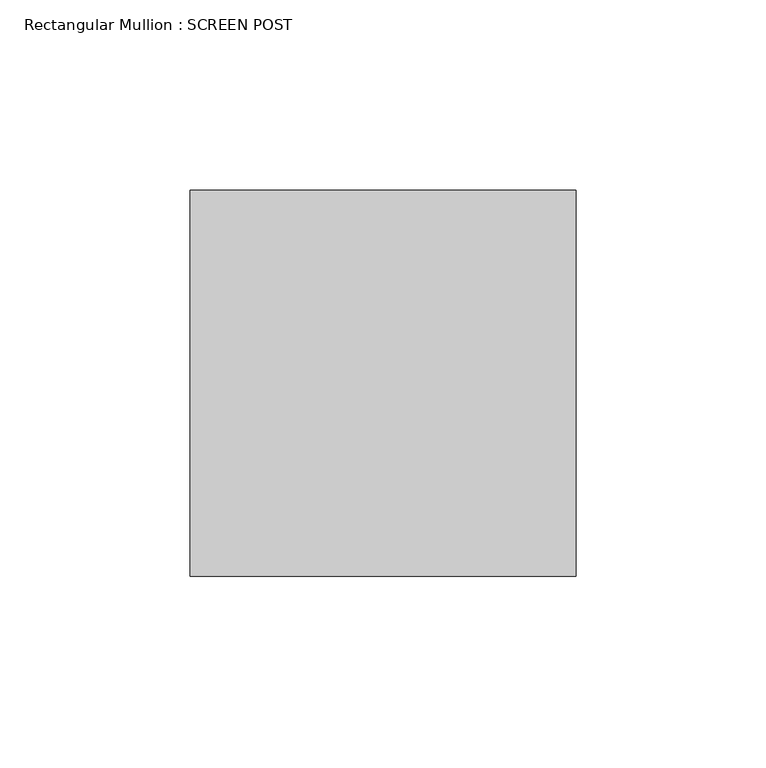
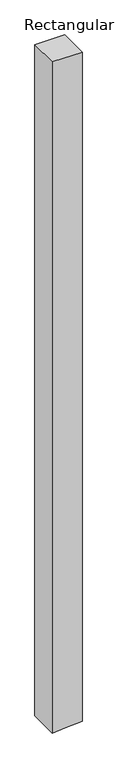
"""IFC4 building model written with IfcOpenShell, lengths in millimetres: member geometry, Rectangular Mullion : SCREEN POST."""

from ifc_helpers import new_model, si_unit, frame, origin, place, context, project, spatial, polyline, outline, extrude, source, transform, mapped, element, save


def rectangular_mullion_screen_post_46a85be0(model_context):
    return source(origin(), model_context, "Body", "SweptSolid", [
        extrude(outline(polyline([(0.0, 50.8), (0.0, -50.8), (-2413.8004128, -50.8), (-2411.021515, -6.3376339), (-2407.4504128, 50.8), (0.0, 50.8)])), frame((0.0, -50.8, 0.0), z_axis=(0.0, 1.0, 0.0), x_axis=(0.0, 0.0, 1.0)), (0.0, 0.0, 1.0), 101.6),
    ])


if __name__ == "__main__":
    model = new_model("IFC4")
    model_context = context("Model", 3, world=origin())
    ifc_project = project(units=[si_unit("LENGTHUNIT", "METRE", prefix="MILLI")], contexts=[model_context])
    site = spatial("IfcSite", under=ifc_project)
    building = spatial("IfcBuilding", under=site)
    placement = place(None, origin())
    rectangular_mullion_screen_post_shape = rectangular_mullion_screen_post_46a85be0(model_context)
    element("IfcMember", 1, ObjectType="Rectangular Mullion : SCREEN POST", at=placement, inside=building, context=model_context, shape_type="MappedRepresentation", body=[
        mapped(rectangular_mullion_screen_post_shape, transform((0.0, 0.0, 0.0), x_axis=(1.0, 0.0, 0.0), y_axis=(0.0, 1.0, 0.0), z_axis=(0.0, 0.0, 1.0))),
    ])
    save(model, "model.ifc")

# Revit data of these elements
# Type "Rectangular Mullion : SCREEN POST"
#   built-in parameter 1007304 = 0.333333 (stored number, unit not read)
#   built-in parameter 1007301 = 0.166667 (stored number, unit not read)
#   built-in parameter 1007300 = 0.166667 (stored number, unit not read)
# Element 1 (IfcMember, "Rectangular Mullion : SCREEN POST")
#   Materials on its faces: "GLULAMS COLUMNS\n(PRESSURE TREATED W/ PENTA IN SOLVENT) (EXTERIOR STAIN: PENOFIN VERDE EXT. STAIN - COLOR: CEDAR)"
# Materials
#   "GLULAMS COLUMNS\n(PRESSURE TREATED W/ PENTA IN SOLVENT) (EXTERIOR STAIN: PENOFIN VERDE EXT. STAIN - COLOR: CEDAR)": class "Wood", colour RGB 164 134 123, transparency 0, Description = "Pinus Echinata", Cost = 0
